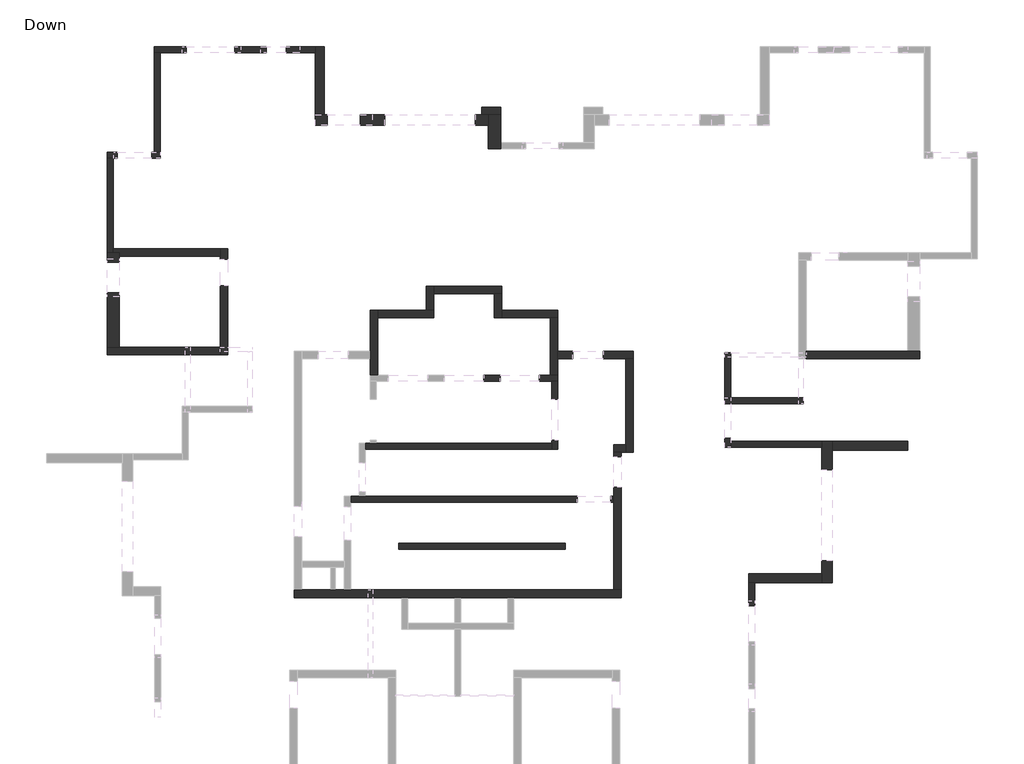
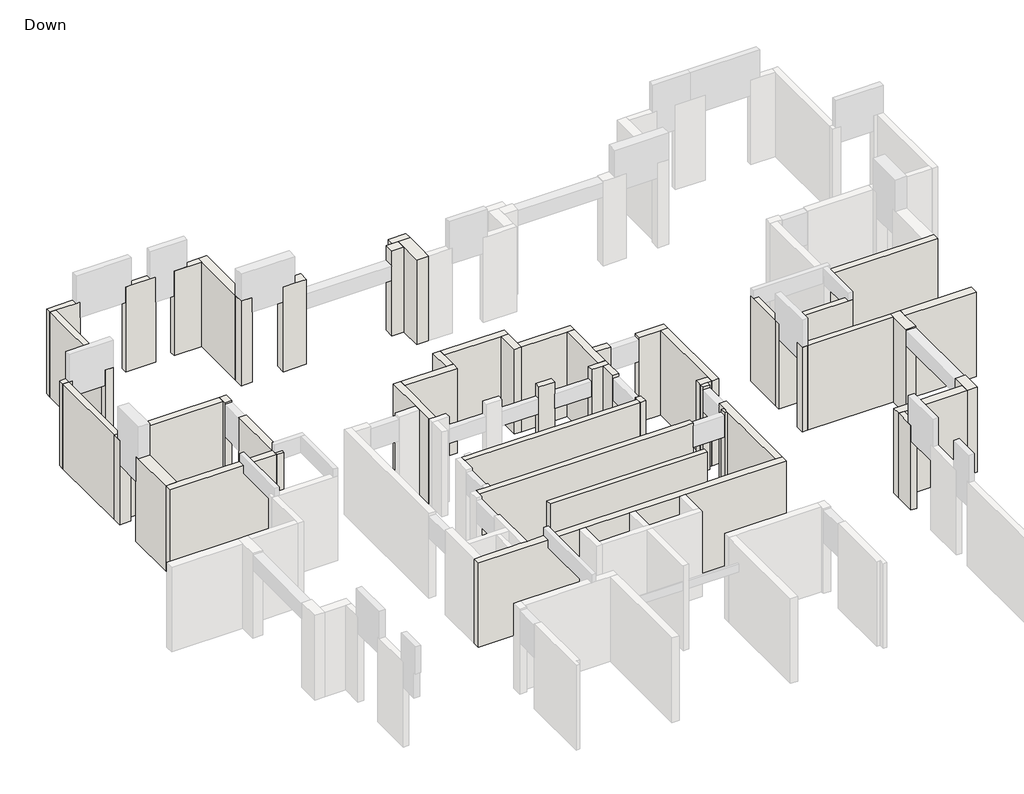
# One storey, part 2 of 3: 51 walls.
# Revit data of these elements (continued)
# Element 18 (IfcWall, "20")
#   Comments = ""
#   Mark = "W64"
#   SOFiSTiK_EdgeZones = "W64"
#   SOFiSTiK_AMG_Comments = ""
#   Top Offset = 0 cm
#   Base Offset = 0 cm
#   wall height = 315 cm
#   SOFiSTiK_AMG_Scheduled = yes
#   SOFiSTiK_AMG_Adjusted = yes
#   Phase Created = New Construction
#   Base Constraint = Down
#   Top Constraint = Typical Floor
#   Materials on its faces: "Concrete"
# Element 19 (IfcWall, "20")
#   Comments = ""
#   Mark = "W70"
#   SOFiSTiK_EdgeZones = "W70"
#   SOFiSTiK_AMG_Comments = ""
#   Top Offset = 0 cm
#   Base Offset = 0 cm
#   wall height = 315 cm
#   SOFiSTiK_AMG_Scheduled = yes
#   SOFiSTiK_AMG_Adjusted = yes
#   Phase Created = New Construction
#   Base Constraint = Down
#   Top Constraint = Typical Floor
#   Materials on its faces: "Concrete"
# Element 20 (IfcWall, "20")
#   Comments = ""
#   Mark = "W74"
#   SOFiSTiK_EdgeZones = "W74"
#   SOFiSTiK_AMG_Comments = ""
#   Top Offset = 0 cm
#   Base Offset = 0 cm
#   wall height = 315 cm
#   SOFiSTiK_AMG_Scheduled = yes
#   SOFiSTiK_AMG_Adjusted = yes
#   Phase Created = New Construction
#   Base Constraint = Down
#   Top Constraint = Typical Floor
#   Materials on its faces: "Concrete"
# Element 21 (IfcWall, "25")
#   Comments = ""
#   Mark = "W81"
#   SOFiSTiK_EdgeZones = "W81"
#   SOFiSTiK_AMG_Comments = ""
#   Top Offset = 0 cm
#   Base Offset = 0 cm
#   wall height = 315 cm
#   SOFiSTiK_AMG_Scheduled = yes
#   SOFiSTiK_AMG_Adjusted = yes
#   Phase Created = New Construction
#   Base Constraint = Down
#   Top Constraint = Typical Floor
#   Materials on its faces: "Concrete"
# Element 22 (IfcWall, "25")
#   Comments = ""
#   Mark = "W82"
#   SOFiSTiK_EdgeZones = "W82"
#   SOFiSTiK_AMG_Comments = ""
#   Top Offset = 0 cm
#   Base Offset = 0 cm
#   wall height = 315 cm
#   SOFiSTiK_AMG_Scheduled = yes
#   SOFiSTiK_AMG_Adjusted = yes
#   Phase Created = New Construction
#   Base Constraint = Down
#   Top Constraint = Typical Floor
#   Materials on its faces: "Concrete"
# Element 23 (IfcWall, "25")
#   Comments = ""
#   Mark = "W83"
#   SOFiSTiK_EdgeZones = "W83"
#   SOFiSTiK_AMG_Comments = ""
#   Top Offset = 0 cm
#   Base Offset = 0 cm
#   wall height = 315 cm
#   SOFiSTiK_AMG_Scheduled = yes
#   SOFiSTiK_AMG_Adjusted = yes
#   Phase Created = New Construction
#   Base Constraint = Down
#   Top Constraint = Typical Floor
#   Materials on its faces: "Concrete"
# Element 24 (IfcWall, "25")
#   Comments = ""
#   Mark = "W84"
#   SOFiSTiK_EdgeZones = "W84"
#   SOFiSTiK_AMG_Comments = ""
#   Top Offset = 0 cm
#   Base Offset = 0 cm
#   wall height = 315 cm
#   SOFiSTiK_AMG_Scheduled = yes
#   SOFiSTiK_AMG_Adjusted = yes
#   Phase Created = New Construction
#   Base Constraint = Down
#   Top Constraint = Typical Floor
#   Materials on its faces: "Concrete"
# Element 25 (IfcWall, "25")
#   Comments = ""
#   Mark = "W89"
#   SOFiSTiK_EdgeZones = "W89"
#   SOFiSTiK_AMG_Comments = ""
#   Top Offset = 0 cm
#   Base Offset = 0 cm
#   wall height = 315 cm
#   SOFiSTiK_AMG_Scheduled = yes
#   SOFiSTiK_AMG_Adjusted = yes
#   Phase Created = New Construction
#   Base Constraint = Down
#   Top Constraint = Typical Floor
#   Materials on its faces: "Concrete"
# Element 26 (IfcWall, "25")
#   Comments = ""
#   Mark = "W98"
#   SOFiSTiK_EdgeZones = "W98"
#   SOFiSTiK_AMG_Comments = ""
#   Top Offset = 0 cm
#   Base Offset = 0 cm
#   wall height = 315 cm
#   SOFiSTiK_AMG_Scheduled = yes
#   SOFiSTiK_AMG_Adjusted = yes
#   Phase Created = New Construction
#   Base Constraint = Down
#   Top Constraint = Typical Floor
#   Materials on its faces: "Concrete"
# Element 27 (IfcWall, "25")
#   Comments = ""
#   Mark = "W99"
#   SOFiSTiK_EdgeZones = "W99"
#   SOFiSTiK_AMG_Comments = ""
#   Top Offset = 0 cm
#   Base Offset = 0 cm
#   wall height = 315 cm
#   SOFiSTiK_AMG_Scheduled = yes
#   SOFiSTiK_AMG_Adjusted = yes
#   Phase Created = New Construction
#   Base Constraint = Down
#   Top Constraint = Typical Floor
#   Materials on its faces: "Concrete"
# Element 28 (IfcWall, "25")
#   Comments = ""
#   Mark = "W104"
#   SOFiSTiK_EdgeZones = "W104"
#   SOFiSTiK_AMG_Comments = ""
#   Top Offset = 0 cm
#   Base Offset = 0 cm
#   wall height = 315 cm
#   SOFiSTiK_AMG_Scheduled = yes
#   SOFiSTiK_AMG_Adjusted = yes
#   Phase Created = New Construction
#   Base Constraint = Down
#   Top Constraint = Typical Floor
#   Materials on its faces: "Concrete"
# Element 29 (IfcWall, "25")
#   Comments = ""
#   Mark = "W105"
#   SOFiSTiK_EdgeZones = "W105"
#   SOFiSTiK_AMG_Comments = ""
#   Top Offset = 0 cm
#   Base Offset = 0 cm
#   wall height = 315 cm
#   SOFiSTiK_AMG_Scheduled = yes
#   SOFiSTiK_AMG_Adjusted = yes
#   Phase Created = New Construction
#   Base Constraint = Down
#   Top Constraint = Typical Floor
#   Materials on its faces: "Concrete"
# Element 30 (IfcWall, "25")
#   Comments = ""
#   Mark = "W106"
#   SOFiSTiK_EdgeZones = "W106"
#   SOFiSTiK_AMG_Comments = ""
#   Top Offset = 0 cm
#   Base Offset = 0 cm
#   wall height = 315 cm
#   SOFiSTiK_AMG_Scheduled = yes
#   SOFiSTiK_AMG_Adjusted = yes
#   Phase Created = New Construction
#   Base Constraint = Down
#   Top Constraint = Typical Floor
#   Materials on its faces: "Concrete"
# Element 31 (IfcWall, "25")
#   Comments = ""
#   Mark = "W107"
#   SOFiSTiK_EdgeZones = "W107"
#   SOFiSTiK_AMG_Comments = ""
#   Top Offset = 0 cm
#   Base Offset = 0 cm
#   wall height = 315 cm
#   SOFiSTiK_AMG_Scheduled = yes
#   SOFiSTiK_AMG_Adjusted = yes
#   Phase Created = New Construction
#   Base Constraint = Down
#   Top Constraint = Typical Floor
#   Materials on its faces: "Concrete"
# Element 32 (IfcWall, "25")
#   Comments = ""
#   Mark = "W108"
#   SOFiSTiK_EdgeZones = "W108"
#   SOFiSTiK_AMG_Comments = ""
#   Top Offset = 0 cm
#   Base Offset = 0 cm
#   wall height = 315 cm
#   SOFiSTiK_AMG_Scheduled = yes
#   SOFiSTiK_AMG_Adjusted = yes
#   Phase Created = New Construction
#   Base Constraint = Down
#   Top Constraint = Typical Floor
#   Materials on its faces: "Concrete"
# Element 33 (IfcWall, "25")
#   Comments = ""
#   Mark = "W109"
#   SOFiSTiK_EdgeZones = "W109"
#   SOFiSTiK_AMG_Comments = ""
#   Top Offset = 0 cm
#   Base Offset = 0 cm
#   wall height = 315 cm
#   SOFiSTiK_AMG_Scheduled = yes
#   SOFiSTiK_AMG_Adjusted = yes
#   Phase Created = New Construction
#   Base Constraint = Down
#   Top Constraint = Typical Floor
#   Materials on its faces: "Concrete"
# Element 34 (IfcWall, "25")
#   Comments = ""
#   Mark = "W110"
#   SOFiSTiK_EdgeZones = "W110"
#   SOFiSTiK_AMG_Comments = ""
#   Top Offset = 0 cm
#   Base Offset = 0 cm
#   wall height = 315 cm
#   SOFiSTiK_AMG_Scheduled = yes
#   SOFiSTiK_AMG_Adjusted = yes
#   Phase Created = New Construction
#   Base Constraint = Down
#   Top Constraint = Typical Floor
#   Materials on its faces: "Concrete"
# Element 35 (IfcWall, "25")
#   Comments = ""
#   Mark = "W111"
#   SOFiSTiK_EdgeZones = "W111"
#   SOFiSTiK_AMG_Comments = ""
#   Top Offset = 0 cm
#   Base Offset = 0 cm
#   wall height = 315 cm
#   SOFiSTiK_AMG_Scheduled = yes
#   SOFiSTiK_AMG_Adjusted = yes
#   Phase Created = New Construction
#   Base Constraint = Down
#   Top Constraint = Typical Floor
#   Materials on its faces: "Concrete"
# Element 36 (IfcWall, "25")
#   Comments = ""
#   Mark = "W112"
#   SOFiSTiK_EdgeZones = "W112"
#   SOFiSTiK_AMG_Comments = ""
#   Top Offset = 0 cm
#   Base Offset = 0 cm
#   wall height = 315 cm
#   SOFiSTiK_AMG_Scheduled = yes
#   SOFiSTiK_AMG_Adjusted = yes
#   Phase Created = New Construction
#   Base Constraint = Down
#   Top Constraint = Typical Floor
#   Materials on its faces: "Concrete"
# Element 37 (IfcWall, "25")
#   Comments = ""
#   Mark = "W113"
#   SOFiSTiK_EdgeZones = "W113"
#   SOFiSTiK_AMG_Comments = ""
#   Top Offset = 0 cm
#   Base Offset = 0 cm
#   wall height = 315 cm
#   SOFiSTiK_AMG_Scheduled = yes
#   SOFiSTiK_AMG_Adjusted = yes
#   Phase Created = New Construction
#   Base Constraint = Down
#   Top Constraint = Typical Floor
#   Materials on its faces: "Concrete"
# Element 38 (IfcWall, "25")
#   Comments = ""
#   Mark = "W114"
#   SOFiSTiK_EdgeZones = "W114"
#   SOFiSTiK_AMG_Comments = ""
#   Top Offset = 0 cm
#   Base Offset = 0 cm
#   wall height = 315 cm
#   SOFiSTiK_AMG_Scheduled = yes
#   SOFiSTiK_AMG_Adjusted = yes
#   Phase Created = New Construction
#   Base Constraint = Down
#   Top Constraint = Typical Floor
#   Materials on its faces: "Concrete"
# Element 39 (IfcWall, "25")
#   Comments = ""
#   Mark = "W115"
#   SOFiSTiK_EdgeZones = "W115"
#   SOFiSTiK_AMG_Comments = "Too Short /"
#   Top Offset = 0 cm
#   Base Offset = 0 cm
#   wall height = 315 cm
#   SOFiSTiK_AMG_Scheduled = yes
#   SOFiSTiK_AMG_Adjusted = yes
#   Phase Created = New Construction
#   Base Constraint = Down
#   Top Constraint = Typical Floor
#   Materials on its faces: "Concrete"
# Element 40 (IfcWall, "30")
#   Comments = ""
#   Mark = "W75"
#   SOFiSTiK_EdgeZones = "W75"
#   SOFiSTiK_AMG_Comments = ""
#   Top Offset = 0 cm
#   Base Offset = 0 cm
#   wall height = 315 cm
#   SOFiSTiK_AMG_Scheduled = yes
#   SOFiSTiK_AMG_Adjusted = yes
#   Phase Created = New Construction
#   Base Constraint = Down
#   Top Constraint = Typical Floor
#   Materials on its faces: "Concrete"
# Element 41 (IfcWall, "30")
#   Comments = ""
#   Mark = "W79"
#   SOFiSTiK_EdgeZones = "W79"
#   SOFiSTiK_AMG_Comments = ""
#   Top Offset = 0 cm
#   Base Offset = 0 cm
#   wall height = 315 cm
#   SOFiSTiK_AMG_Scheduled = yes
#   SOFiSTiK_AMG_Adjusted = yes
#   Phase Created = New Construction
#   Base Constraint = Down
#   Top Constraint = Typical Floor
#   Materials on its faces: "Concrete"
# Element 42 (IfcWall, "30")
#   Comments = ""
#   Mark = "W80"
#   SOFiSTiK_EdgeZones = "W80"
#   SOFiSTiK_AMG_Comments = ""
#   Top Offset = 0 cm
#   Base Offset = 0 cm
#   wall height = 315 cm
#   SOFiSTiK_AMG_Scheduled = yes
#   SOFiSTiK_AMG_Adjusted = yes
#   Phase Created = New Construction
#   Base Constraint = Down
#   Top Constraint = Typical Floor
#   Materials on its faces: "Concrete"
# Element 43 (IfcWall, "35")
#   Comments = ""
#   Mark = "W1"
#   SOFiSTiK_EdgeZones = "W1"
#   SOFiSTiK_AMG_Comments = ""
#   Top Offset = 0 cm
#   Base Offset = 0 cm
#   wall height = 315 cm
#   SOFiSTiK_AMG_Scheduled = yes
#   SOFiSTiK_AMG_Adjusted = yes
#   Phase Created = New Construction
#   Base Constraint = Down
#   Top Constraint = Typical Floor
#   Materials on its faces: "Concrete"
# Element 44 (IfcWall, "35")
#   Comments = ""
#   Mark = "W2"
#   SOFiSTiK_EdgeZones = "W2"
#   SOFiSTiK_AMG_Comments = ""
#   Top Offset = 0 cm
#   Base Offset = 0 cm
#   wall height = 315 cm
#   SOFiSTiK_AMG_Scheduled = yes
#   SOFiSTiK_AMG_Adjusted = yes
#   Phase Created = New Construction
#   Base Constraint = Down
#   Top Constraint = Typical Floor
#   Materials on its faces: "Concrete"
# Element 45 (IfcWall, "35")
#   Comments = ""
#   Mark = "W3"
#   SOFiSTiK_EdgeZones = "W3"
#   SOFiSTiK_AMG_Comments = ""
#   Top Offset = 0 cm
#   Base Offset = 0 cm
#   wall height = 315 cm
#   SOFiSTiK_AMG_Scheduled = yes
#   SOFiSTiK_AMG_Adjusted = yes
#   Phase Created = New Construction
#   Base Constraint = Down
#   Top Constraint = Typical Floor
#   Materials on its faces: "Concrete"
# Element 46 (IfcWall, "35")
#   Comments = ""
#   Mark = "W4"
#   SOFiSTiK_EdgeZones = "W4"
#   SOFiSTiK_AMG_Comments = ""
#   Top Offset = 0 cm
#   Base Offset = 0 cm
#   wall height = 315 cm
#   SOFiSTiK_AMG_Scheduled = yes
#   SOFiSTiK_AMG_Adjusted = yes
#   Phase Created = New Construction
#   Base Constraint = Down
#   Top Constraint = Typical Floor
#   Materials on its faces: "Concrete"
# Element 47 (IfcWall, "35")
#   Comments = ""
#   Mark = "W11"
#   SOFiSTiK_EdgeZones = "W11"
#   SOFiSTiK_AMG_Comments = ""
#   Top Offset = 0 cm
#   Base Offset = 0 cm
#   wall height = 315 cm
#   SOFiSTiK_AMG_Scheduled = yes
#   SOFiSTiK_AMG_Adjusted = yes
#   Phase Created = New Construction
#   Base Constraint = Down
#   Top Constraint = Typical Floor
#   Materials on its faces: "Concrete"
# Element 48 (IfcWall, "35")
#   Comments = ""
#   Mark = "W12"
#   SOFiSTiK_EdgeZones = "W12"
#   SOFiSTiK_AMG_Comments = ""
#   Top Offset = 0 cm
#   Base Offset = 0 cm
#   wall height = 315 cm
#   SOFiSTiK_AMG_Scheduled = yes
#   SOFiSTiK_AMG_Adjusted = yes
#   Phase Created = New Construction
#   Base Constraint = Down
#   Top Constraint = Typical Floor
#   Materials on its faces: "Concrete"
# Element 49 (IfcWall, "40")
#   Comments = ""
#   Mark = "W116"
#   SOFiSTiK_EdgeZones = "W116"
#   SOFiSTiK_AMG_Comments = ""
#   Top Offset = 0 cm
#   Base Offset = 0 cm
#   wall height = 315 cm
#   SOFiSTiK_AMG_Scheduled = yes
#   SOFiSTiK_AMG_Adjusted = yes
#   Phase Created = New Construction
#   Base Constraint = Down
#   Top Constraint = Typical Floor
#   Materials on its faces: "Concrete"
# Element 50 (IfcWall, "40")
#   Comments = ""
#   Mark = "W121"
#   SOFiSTiK_EdgeZones = "W121"
#   SOFiSTiK_AMG_Comments = ""
#   Top Offset = 0 cm
#   Base Offset = 0 cm
#   wall height = 315 cm
#   SOFiSTiK_AMG_Scheduled = yes
#   SOFiSTiK_AMG_Adjusted = yes
#   Phase Created = New Construction
#   Base Constraint = Down
#   Top Constraint = Typical Floor
#   Materials on its faces: "Concrete"
# Element 51 (IfcWall, "42")
#   Comments = ""
#   Mark = "W13"
#   SOFiSTiK_EdgeZones = "W13"
#   SOFiSTiK_AMG_Comments = ""
#   Top Offset = 0 cm
#   Base Offset = 0 cm
#   wall height = 315 cm
#   SOFiSTiK_AMG_Scheduled = yes
#   SOFiSTiK_AMG_Adjusted = yes
#   Phase Created = New Construction
#   Base Constraint = Down
#   Top Constraint = Typical Floor
#   Materials on its faces: "Concrete"
# Materials
#   "Concrete": class "Concrete", colour RGB 192 192 192, transparency 0, Keynote = "01000", Description = "Cast-in-place concrete", Cost = 0
